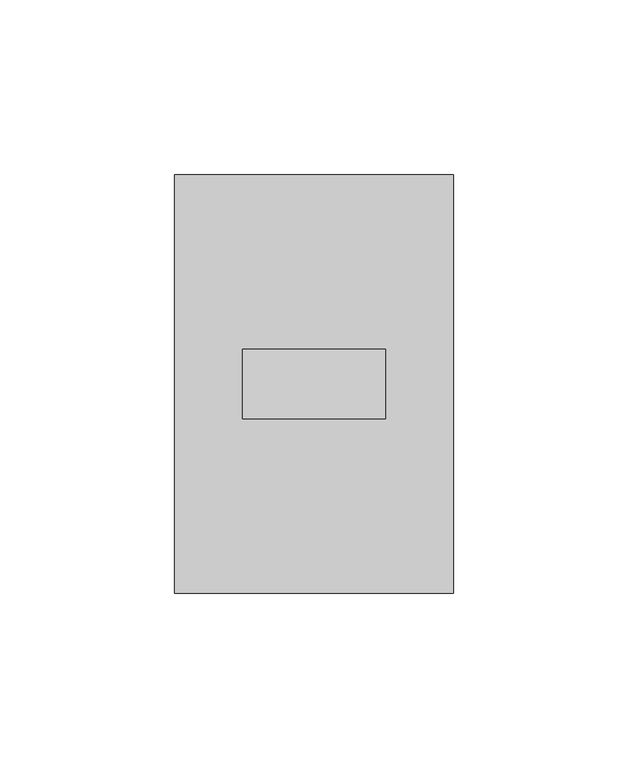
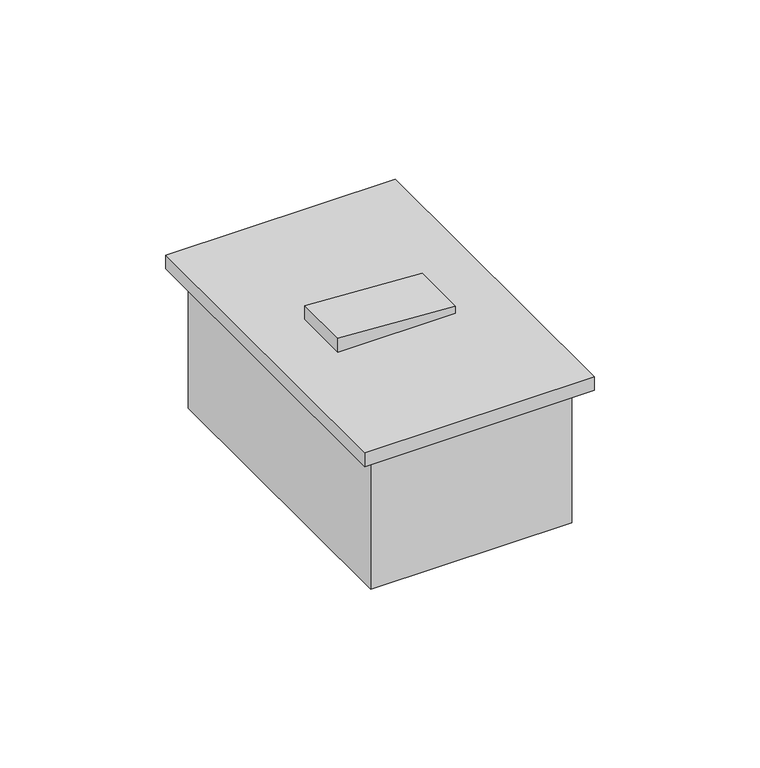
"""IFC4 building model written with IfcOpenShell, lengths in millimetres: proxy geometry, CAIXA VERTICE V7 : Interruptor 1s."""

import ifcopenshell
import ifcopenshell.guid

model = None  # the IFC model being written
_history = None  # IfcOwnerHistory: only IFC2X3 demands one
_inside = {}  # id of a spatial element -> (the spatial element, [elements in it])
_under = {}  # id of a project, library or spatial element -> (it, [spatial elements below it])
_declared = {}  # id of a project -> (the project, [libraries it declares])
_typed = {}  # id of a type object -> (the type object, [elements of that type])
_made_of = {}  # id of a material, layer set ... -> (it, [elements and type objects made of it])


def new_model(schema):
    """Start an empty IFC model of exactly this schema.

    Asked for "IFC4X3", IfcOpenShell would pick the latest addendum, in which some entities
    have other attributes; the version numbers below select the first issue.
    IFC2X3 requires an IfcOwnerHistory on every rooted entity: one is made here for all.
    """
    global model, _history
    if schema == "IFC4X3":
        model = ifcopenshell.file(schema_version=(4, 3, 0, 0))
    else:
        model = ifcopenshell.file(schema=schema)
    _inside.clear()
    _under.clear()
    _declared.clear()
    _typed.clear()
    _made_of.clear()
    _history = None
    if model.schema == "IFC2X3":
        org = make("IfcOrganization", Name="unknown")
        user = make(
            "IfcPersonAndOrganization",
            ThePerson=make("IfcPerson", FamilyName="unknown"),
            TheOrganization=org,
        )
        app = make(
            "IfcApplication",
            ApplicationDeveloper=org,
            Version="unknown",
            ApplicationFullName="unknown",
            ApplicationIdentifier="unknown",
        )
        _history = make(
            "IfcOwnerHistory",
            OwningUser=user,
            OwningApplication=app,
            ChangeAction="ADDED",
            CreationDate=0,
        )
    return model


def make(cls, **values):
    """One entity of the class cls with the attributes given. An attribute that is None is left unset."""
    return model.create_entity(
        cls, **{name: value for name, value in values.items() if value is not None}
    )


def rooted(cls, **values):
    """An entity with a GlobalId (a new one), such as an element, a storey or a relation."""
    return make(cls, GlobalId=ifcopenshell.guid.new(), OwnerHistory=_history, **values)


def si_unit(unit_type, name, prefix=None):
    """IfcSIUnit, for example si_unit("LENGTHUNIT", "METRE", prefix="MILLI")."""
    return make("IfcSIUnit", UnitType=unit_type, Prefix=prefix, Name=name)


def assignment(units):
    """IfcUnitAssignment: the units of a project."""
    return None if units is None else make("IfcUnitAssignment", Units=units)


def point(xyz):
    """IfcCartesianPoint."""
    return None if xyz is None else make("IfcCartesianPoint", Coordinates=xyz)


def direction(xyz):
    """IfcDirection."""
    return None if xyz is None else make("IfcDirection", DirectionRatios=xyz)


def frame(location, z_axis=None, x_axis=None):
    """IfcAxis2Placement3D, a coordinate frame: its origin and axes. An axis left out is left unset."""
    return make(
        "IfcAxis2Placement3D",
        Location=point(location),
        Axis=direction(z_axis),
        RefDirection=direction(x_axis),
    )


def origin():
    """The frame at (0, 0, 0) with its axes left unset."""
    return frame((0.0, 0.0, 0.0))


def origin_with_axes():
    """The frame at (0, 0, 0) with the z axis (0, 0, 1) and the x axis (1, 0, 0) written out."""
    return frame((0.0, 0.0, 0.0), z_axis=(0.0, 0.0, 1.0), x_axis=(1.0, 0.0, 0.0))


def place(relative_to, where):
    """IfcLocalPlacement: puts the frame where relative to a parent placement (None: the world)."""
    return make(
        "IfcLocalPlacement", PlacementRelTo=relative_to, RelativePlacement=where
    )


def context(
    kind, dimensions, precision=None, world=None, true_north=None, identifier=None
):
    """IfcGeometricRepresentationContext, for example the 3D "Model" context."""
    return make(
        "IfcGeometricRepresentationContext",
        ContextIdentifier=identifier,
        ContextType=kind,
        CoordinateSpaceDimension=dimensions,
        Precision=precision,
        WorldCoordinateSystem=world,
        TrueNorth=true_north,
    )


def project(units=None, contexts=None):
    """IfcProject with its units and contexts."""
    return rooted(
        "IfcProject",
        Name="project",
        RepresentationContexts=contexts,
        UnitsInContext=assignment(units),
    )


def spatial(cls, under=None, at=None, **own):
    """A site, building, storey or space (cls), placed at a placement, below another one or the project."""
    s = rooted(cls, ObjectPlacement=at, **own)
    if under is not None:
        _under.setdefault(under.id(), (under, []))[1].append(s)
    return s


def polyline(points):
    """IfcPolyline through the points."""
    return make("IfcPolyline", Points=[point(p) for p in points])


def outline(outer, holes=None, kind="AREA"):
    """IfcArbitraryClosedProfileDef: a profile drawn as a closed curve; with holes, ...WithVoids."""
    if holes is None:
        return make("IfcArbitraryClosedProfileDef", ProfileType=kind, OuterCurve=outer)
    return make(
        "IfcArbitraryProfileDefWithVoids",
        ProfileType=kind,
        OuterCurve=outer,
        InnerCurves=holes,
    )


def extrude(swept, where, along, depth):
    """IfcExtrudedAreaSolid: the profile swept, set in the frame where, extruded along a direction by depth."""
    return make(
        "IfcExtrudedAreaSolid",
        SweptArea=swept,
        Position=where,
        ExtrudedDirection=direction(along),
        Depth=depth,
    )


def faces_of(points, faces, orient=None, outer=None):
    """IfcFace entities. A face is a list of loops; a loop is a list of indices into points, from 0.

    orient and outer hold one flag for each loop. By default every Orientation is true, the
    first loop of a face is its IfcFaceOuterBound and the others are IfcFaceBound.
    """
    made = []
    for i, loops in enumerate(faces):
        bounds = []
        for j, loop in enumerate(loops):
            is_outer = j == 0 if outer is None else outer[i][j]
            bounds.append(
                make(
                    "IfcFaceOuterBound" if is_outer else "IfcFaceBound",
                    Bound=make("IfcPolyLoop", Polygon=[points[k] for k in loop]),
                    Orientation=True if orient is None else orient[i][j],
                )
            )
        made.append(make("IfcFace", Bounds=bounds))
    return made


def faceted_brep(points, faces, orient=None, outer=None, voids=None):
    """IfcFacetedBrep: a solid bounded by flat faces; with voids (closed shells), ...WithVoids."""
    shared = [point(p) for p in points]
    hull = make("IfcClosedShell", CfsFaces=faces_of(shared, faces, orient, outer))
    if voids is None:
        return make("IfcFacetedBrep", Outer=hull)
    return make(
        "IfcFacetedBrepWithVoids",
        Outer=hull,
        Voids=[
            make(cls, CfsFaces=faces_of(shared, fs, o, b)) for cls, fs, o, b in voids
        ],
    )


def shape(context_of_items, identifier, shape_type, items):
    """IfcShapeRepresentation: the items that make up one representation, for example the "Body"."""
    return make(
        "IfcShapeRepresentation",
        ContextOfItems=context_of_items,
        RepresentationIdentifier=identifier,
        RepresentationType=shape_type,
        Items=items,
    )


def source(mapping_origin, context_of_items, identifier, shape_type, items):
    """IfcRepresentationMap: a shape defined once, which mapped items show again and again."""
    return make(
        "IfcRepresentationMap",
        MappingOrigin=mapping_origin,
        MappedRepresentation=shape(context_of_items, identifier, shape_type, items),
    )


def transform(
    local_origin,
    x_axis=None,
    y_axis=None,
    z_axis=None,
    scale=None,
    scale2=None,
    scale3=None,
    uniform=True,
):
    """IfcCartesianTransformationOperator3D, or its non-uniform kind. x_axis, y_axis, z_axis: its Axis1, 2, 3."""
    if uniform:
        return make(
            "IfcCartesianTransformationOperator3D",
            Axis1=direction(x_axis),
            Axis2=direction(y_axis),
            LocalOrigin=point(local_origin),
            Scale=scale,
            Axis3=direction(z_axis),
        )
    return make(
        "IfcCartesianTransformationOperator3DnonUniform",
        Axis1=direction(x_axis),
        Axis2=direction(y_axis),
        LocalOrigin=point(local_origin),
        Scale=scale,
        Axis3=direction(z_axis),
        Scale2=scale2,
        Scale3=scale3,
    )


def mapped(mapping_source, mapping_target):
    """IfcMappedItem: shows the shape of a source again, moved by a transform."""
    return make(
        "IfcMappedItem", MappingSource=mapping_source, MappingTarget=mapping_target
    )


def made_of(thing, what):
    """Note that an element or type object is made of a material, layer set ...; save() writes the relation."""
    if what is not None:
        _made_of.setdefault(what.id(), (what, []))[1].append(thing)
    return thing


def element(
    cls,
    number,
    at=None,
    inside=None,
    cuts=None,
    type_object=None,
    material=None,
    context=None,
    identifier="Body",
    shape_type=None,
    held_by="IfcProductDefinitionShape",
    body=None,
    shapes=None,
    **own,
):
    """One element of the class cls, such as IfcWall. Its Tag is "e" and its number.

    at: its placement. inside: the storey or other place that contains it. cuts: it is an
    opening in that element (IfcRelVoidsElement). A single representation is given by context,
    identifier, shape_type and body (its items); several are given by shapes. held_by: the class
    of the entity that holds the representations. save() writes the other relations.
    """
    e = rooted(cls, Tag="e%d" % number, ObjectPlacement=at, **own)
    if body is not None:
        shapes = [shape(context, identifier, shape_type, body)]
    if shapes is not None:
        e.Representation = make(held_by, Representations=shapes)
    if inside is not None:
        _inside.setdefault(inside.id(), (inside, []))[1].append(e)
    if cuts is not None:
        rooted(
            "IfcRelVoidsElement", RelatingBuildingElement=cuts, RelatedOpeningElement=e
        )
    if type_object is not None:
        _typed.setdefault(type_object.id(), (type_object, []))[1].append(e)
    return made_of(e, material)


def aggregate(whole, parts):
    """IfcRelAggregates: a whole, such as a stair, and the parts it consists of."""
    return rooted("IfcRelAggregates", RelatingObject=whole, RelatedObjects=parts)


def save(model, path):
    """Write the relations noted so far, then the file.

    IfcRelAggregates (storeys below a building ...), IfcRelContainedInSpatialStructure (elements
    in a storey), IfcRelDefinesByType, IfcRelAssociatesMaterial and IfcRelDeclares: one each for
    every whole, place, type object, material and project.
    """
    for whole, parts in _under.values():
        aggregate(whole, parts)
    for where, things in _inside.values():
        rooted(
            "IfcRelContainedInSpatialStructure",
            RelatedElements=things,
            RelatingStructure=where,
        )
    for kind, things in _typed.values():
        rooted("IfcRelDefinesByType", RelatedObjects=things, RelatingType=kind)
    for what, things in _made_of.values():
        rooted("IfcRelAssociatesMaterial", RelatedObjects=things, RelatingMaterial=what)
    for by, libraries in _declared.values():
        rooted("IfcRelDeclares", RelatingContext=by, RelatedDefinitions=libraries)
    model.write(path)


def electrical_fixtures_62d980e5(model_context):
    return source(origin(), model_context, "Body", "SolidModel", [
        extrude(outline(polyline([(5.0, 20.5), (7.5, 20.5), (10.0, -20.5), (5.0, -20.5), (5.0, 20.5)])), frame((0.0, 1090.0, 0.0), z_axis=(0.0, 1.0, 0.0), x_axis=(0.0, 0.0, 1.0)), (0.0, 0.0, 1.0), 20.0),
        faceted_brep([(35.0, 1155.0, 0.0), (-35.0, 1155.0, 0.0), (-35.0, 1045.0, 0.0), (35.0, 1045.0, 0.0), (33.0, 1153.0, 0.0), (33.0, 1047.0, 0.0), (-33.0, 1047.0, 0.0), (-33.0, 1153.0, 0.0), (33.0, 1047.0, -48.0), (33.0, 1153.0, -48.0), (-33.0, 1153.0, -48.0), (-33.0, 1047.0, -48.0), (35.0, 1155.0, -50.0), (35.0, 1045.0, -50.0), (-35.0, 1045.0, -50.0), (-35.0, 1155.0, -50.0)], [[[0, 1, 2, 3], [4, 5, 6, 7]], [[8, 9, 10, 11]], [[12, 13, 14, 15]], [[12, 15, 1, 0]], [[1, 15, 14, 2]], [[2, 14, 13, 3]], [[3, 13, 12, 0]], [[5, 4, 9, 8]], [[6, 5, 8, 11]], [[7, 6, 11, 10]], [[4, 7, 10, 9]]]),
        extrude(outline(polyline([(40.0, 1160.0), (40.0, 1040.0), (-40.0, 1040.0), (-40.0, 1160.0), (40.0, 1160.0)])), origin_with_axes(), (0.0, 0.0, 1.0), 5.0),
    ])


if __name__ == "__main__":
    model = new_model("IFC4")
    model_context = context("Model", 3, world=origin())
    ifc_project = project(units=[si_unit("LENGTHUNIT", "METRE", prefix="MILLI")], contexts=[model_context])
    site = spatial("IfcSite", under=ifc_project)
    building = spatial("IfcBuilding", under=site)
    placement = place(None, origin())
    electrical_fixtures_shape = electrical_fixtures_62d980e5(model_context)
    element("IfcBuildingElementProxy", 1, Name="CAIXA VERTICE V7 : Interruptor 1s", ObjectType="CAIXA VERTICE V7 : Interruptor 1s", at=placement, inside=building, context=model_context, shape_type="MappedRepresentation", body=[
        mapped(electrical_fixtures_shape, transform((0.0, 0.0, 0.0), x_axis=(1.0, 0.0, 0.0), y_axis=(0.0, 1.0, 0.0), z_axis=(0.0, 0.0, 1.0))),
    ])
    save(model, "model.ifc")

# Revit data of these elements
# Type "CAIXA VERTICE V7 : Interruptor 1s"
#   URL = "www.facebook.com/verticetreinamentos"
#   SEÇÃO [instance default] = ""
#   Rotação [instance default] = 0.00°
#   LARGURA DA TAMPA = 0.08 m
#   BORDA = 0.01 m
#   ALTURA DE INSTALAÇÃO [instance default] = 1.10 m
#   Distância Anotação [instance default] = 0.0015 m
#   ALTURA DA TAMPA = 0.12 m
#   Vertical [instance default] = yes
#   VER SEÇÃO [instance default] = yes
#   SHADE ESQ [instance default] = no
#   SHADE DIR [instance default] = yes
#   HORIZONTAL [instance default] = no
#   ANDAR COM A LEGENDA [instance default] = 0
#   Material Tampa [instance default] = Plástico, branco opaco
#   Caixa = element 1798509
#   Anotação = element 1798523
#   Default Elevation = 0
# Element 1 (IfcBuildingElementProxy, "CAIXA VERTICE V7 : Interruptor 1s")
#   SEÇÃO = "1"
#   Materials on its faces: "Plástico, branco opaco"
# Materials
#   "Plástico, branco opaco": class "Plástico", colour RGB 120 120 120, transparency 0, Description = "Plastic, generic, opaque white", Cost = 0
